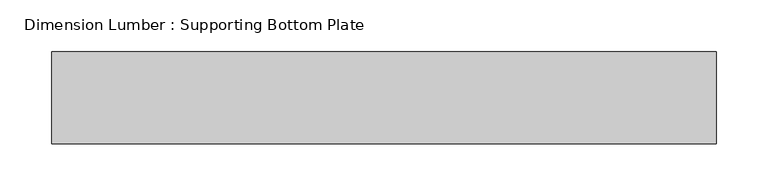
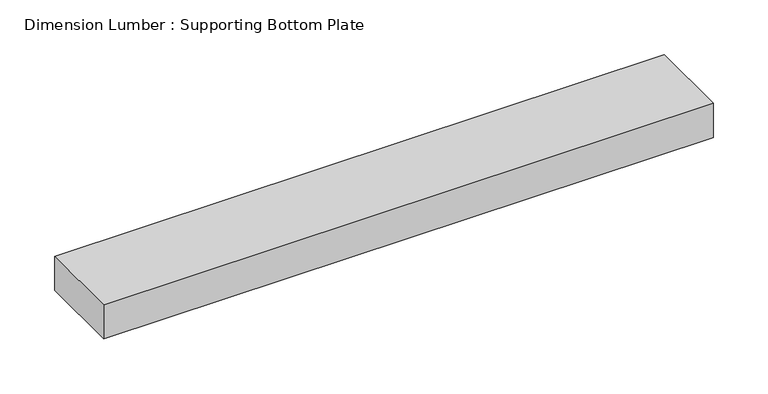
"""IFC4 building model written with IfcOpenShell, lengths in millimetres: beam geometry, Dimension Lumber : Supporting Bottom Plate."""

import ifcopenshell
import ifcopenshell.guid

model = None  # the IFC model being written
_history = None  # IfcOwnerHistory: only IFC2X3 demands one
_inside = {}  # id of a spatial element -> (the spatial element, [elements in it])
_under = {}  # id of a project, library or spatial element -> (it, [spatial elements below it])
_declared = {}  # id of a project -> (the project, [libraries it declares])
_typed = {}  # id of a type object -> (the type object, [elements of that type])
_made_of = {}  # id of a material, layer set ... -> (it, [elements and type objects made of it])


def new_model(schema):
    """Start an empty IFC model of exactly this schema.

    Asked for "IFC4X3", IfcOpenShell would pick the latest addendum, in which some entities
    have other attributes; the version numbers below select the first issue.
    IFC2X3 requires an IfcOwnerHistory on every rooted entity: one is made here for all.
    """
    global model, _history
    if schema == "IFC4X3":
        model = ifcopenshell.file(schema_version=(4, 3, 0, 0))
    else:
        model = ifcopenshell.file(schema=schema)
    _inside.clear()
    _under.clear()
    _declared.clear()
    _typed.clear()
    _made_of.clear()
    _history = None
    if model.schema == "IFC2X3":
        org = make("IfcOrganization", Name="unknown")
        user = make(
            "IfcPersonAndOrganization",
            ThePerson=make("IfcPerson", FamilyName="unknown"),
            TheOrganization=org,
        )
        app = make(
            "IfcApplication",
            ApplicationDeveloper=org,
            Version="unknown",
            ApplicationFullName="unknown",
            ApplicationIdentifier="unknown",
        )
        _history = make(
            "IfcOwnerHistory",
            OwningUser=user,
            OwningApplication=app,
            ChangeAction="ADDED",
            CreationDate=0,
        )
    return model


def make(cls, **values):
    """One entity of the class cls with the attributes given. An attribute that is None is left unset."""
    return model.create_entity(
        cls, **{name: value for name, value in values.items() if value is not None}
    )


def rooted(cls, **values):
    """An entity with a GlobalId (a new one), such as an element, a storey or a relation."""
    return make(cls, GlobalId=ifcopenshell.guid.new(), OwnerHistory=_history, **values)


def si_unit(unit_type, name, prefix=None):
    """IfcSIUnit, for example si_unit("LENGTHUNIT", "METRE", prefix="MILLI")."""
    return make("IfcSIUnit", UnitType=unit_type, Prefix=prefix, Name=name)


def assignment(units):
    """IfcUnitAssignment: the units of a project."""
    return None if units is None else make("IfcUnitAssignment", Units=units)


def point(xyz):
    """IfcCartesianPoint."""
    return None if xyz is None else make("IfcCartesianPoint", Coordinates=xyz)


def direction(xyz):
    """IfcDirection."""
    return None if xyz is None else make("IfcDirection", DirectionRatios=xyz)


def frame(location, z_axis=None, x_axis=None):
    """IfcAxis2Placement3D, a coordinate frame: its origin and axes. An axis left out is left unset."""
    return make(
        "IfcAxis2Placement3D",
        Location=point(location),
        Axis=direction(z_axis),
        RefDirection=direction(x_axis),
    )


def origin():
    """The frame at (0, 0, 0) with its axes left unset."""
    return frame((0.0, 0.0, 0.0))


def place(relative_to, where):
    """IfcLocalPlacement: puts the frame where relative to a parent placement (None: the world)."""
    return make(
        "IfcLocalPlacement", PlacementRelTo=relative_to, RelativePlacement=where
    )


def context(
    kind, dimensions, precision=None, world=None, true_north=None, identifier=None
):
    """IfcGeometricRepresentationContext, for example the 3D "Model" context."""
    return make(
        "IfcGeometricRepresentationContext",
        ContextIdentifier=identifier,
        ContextType=kind,
        CoordinateSpaceDimension=dimensions,
        Precision=precision,
        WorldCoordinateSystem=world,
        TrueNorth=true_north,
    )


def project(units=None, contexts=None):
    """IfcProject with its units and contexts."""
    return rooted(
        "IfcProject",
        Name="project",
        RepresentationContexts=contexts,
        UnitsInContext=assignment(units),
    )


def spatial(cls, under=None, at=None, **own):
    """A site, building, storey or space (cls), placed at a placement, below another one or the project."""
    s = rooted(cls, ObjectPlacement=at, **own)
    if under is not None:
        _under.setdefault(under.id(), (under, []))[1].append(s)
    return s


def polyline(points):
    """IfcPolyline through the points."""
    return make("IfcPolyline", Points=[point(p) for p in points])


def outline(outer, holes=None, kind="AREA"):
    """IfcArbitraryClosedProfileDef: a profile drawn as a closed curve; with holes, ...WithVoids."""
    if holes is None:
        return make("IfcArbitraryClosedProfileDef", ProfileType=kind, OuterCurve=outer)
    return make(
        "IfcArbitraryProfileDefWithVoids",
        ProfileType=kind,
        OuterCurve=outer,
        InnerCurves=holes,
    )


def extrude(swept, where, along, depth):
    """IfcExtrudedAreaSolid: the profile swept, set in the frame where, extruded along a direction by depth."""
    return make(
        "IfcExtrudedAreaSolid",
        SweptArea=swept,
        Position=where,
        ExtrudedDirection=direction(along),
        Depth=depth,
    )


def shape(context_of_items, identifier, shape_type, items):
    """IfcShapeRepresentation: the items that make up one representation, for example the "Body"."""
    return make(
        "IfcShapeRepresentation",
        ContextOfItems=context_of_items,
        RepresentationIdentifier=identifier,
        RepresentationType=shape_type,
        Items=items,
    )


def source(mapping_origin, context_of_items, identifier, shape_type, items):
    """IfcRepresentationMap: a shape defined once, which mapped items show again and again."""
    return make(
        "IfcRepresentationMap",
        MappingOrigin=mapping_origin,
        MappedRepresentation=shape(context_of_items, identifier, shape_type, items),
    )


def transform(
    local_origin,
    x_axis=None,
    y_axis=None,
    z_axis=None,
    scale=None,
    scale2=None,
    scale3=None,
    uniform=True,
):
    """IfcCartesianTransformationOperator3D, or its non-uniform kind. x_axis, y_axis, z_axis: its Axis1, 2, 3."""
    if uniform:
        return make(
            "IfcCartesianTransformationOperator3D",
            Axis1=direction(x_axis),
            Axis2=direction(y_axis),
            LocalOrigin=point(local_origin),
            Scale=scale,
            Axis3=direction(z_axis),
        )
    return make(
        "IfcCartesianTransformationOperator3DnonUniform",
        Axis1=direction(x_axis),
        Axis2=direction(y_axis),
        LocalOrigin=point(local_origin),
        Scale=scale,
        Axis3=direction(z_axis),
        Scale2=scale2,
        Scale3=scale3,
    )


def mapped(mapping_source, mapping_target):
    """IfcMappedItem: shows the shape of a source again, moved by a transform."""
    return make(
        "IfcMappedItem", MappingSource=mapping_source, MappingTarget=mapping_target
    )


def made_of(thing, what):
    """Note that an element or type object is made of a material, layer set ...; save() writes the relation."""
    if what is not None:
        _made_of.setdefault(what.id(), (what, []))[1].append(thing)
    return thing


def element(
    cls,
    number,
    at=None,
    inside=None,
    cuts=None,
    type_object=None,
    material=None,
    context=None,
    identifier="Body",
    shape_type=None,
    held_by="IfcProductDefinitionShape",
    body=None,
    shapes=None,
    **own,
):
    """One element of the class cls, such as IfcWall. Its Tag is "e" and its number.

    at: its placement. inside: the storey or other place that contains it. cuts: it is an
    opening in that element (IfcRelVoidsElement). A single representation is given by context,
    identifier, shape_type and body (its items); several are given by shapes. held_by: the class
    of the entity that holds the representations. save() writes the other relations.
    """
    e = rooted(cls, Tag="e%d" % number, ObjectPlacement=at, **own)
    if body is not None:
        shapes = [shape(context, identifier, shape_type, body)]
    if shapes is not None:
        e.Representation = make(held_by, Representations=shapes)
    if inside is not None:
        _inside.setdefault(inside.id(), (inside, []))[1].append(e)
    if cuts is not None:
        rooted(
            "IfcRelVoidsElement", RelatingBuildingElement=cuts, RelatedOpeningElement=e
        )
    if type_object is not None:
        _typed.setdefault(type_object.id(), (type_object, []))[1].append(e)
    return made_of(e, material)


def aggregate(whole, parts):
    """IfcRelAggregates: a whole, such as a stair, and the parts it consists of."""
    return rooted("IfcRelAggregates", RelatingObject=whole, RelatedObjects=parts)


def save(model, path):
    """Write the relations noted so far, then the file.

    IfcRelAggregates (storeys below a building ...), IfcRelContainedInSpatialStructure (elements
    in a storey), IfcRelDefinesByType, IfcRelAssociatesMaterial and IfcRelDeclares: one each for
    every whole, place, type object, material and project.
    """
    for whole, parts in _under.values():
        aggregate(whole, parts)
    for where, things in _inside.values():
        rooted(
            "IfcRelContainedInSpatialStructure",
            RelatedElements=things,
            RelatingStructure=where,
        )
    for kind, things in _typed.values():
        rooted("IfcRelDefinesByType", RelatedObjects=things, RelatingType=kind)
    for what, things in _made_of.values():
        rooted("IfcRelAssociatesMaterial", RelatedObjects=things, RelatingMaterial=what)
    for by, libraries in _declared.values():
        rooted("IfcRelDeclares", RelatingContext=by, RelatedDefinitions=libraries)
    model.write(path)


def dimension_lumber_supporting_bottom_plate_50cface6(model_context):
    return source(origin(), model_context, "Body", "SweptSolid", [
        extrude(outline(polyline([(320.675, 44.45), (320.675, -44.45), (-320.675, -44.45), (-320.675, 44.45), (320.675, 44.45)])), frame((0.0, 0.0, -19.05), z_axis=(0.0, 0.0, 1.0), x_axis=(1.0, 0.0, 0.0)), (0.0, 0.0, 1.0), 38.1),
    ])


if __name__ == "__main__":
    model = new_model("IFC4")
    model_context = context("Model", 3, world=origin())
    ifc_project = project(units=[si_unit("LENGTHUNIT", "METRE", prefix="MILLI")], contexts=[model_context])
    site = spatial("IfcSite", under=ifc_project)
    building = spatial("IfcBuilding", under=site)
    placement = place(None, origin())
    dimension_lumber_supporting_bottom_plate_shape = dimension_lumber_supporting_bottom_plate_50cface6(model_context)
    element("IfcBeam", 1, ObjectType="Dimension Lumber : Supporting Bottom Plate", at=placement, inside=building, context=model_context, shape_type="MappedRepresentation", body=[
        mapped(dimension_lumber_supporting_bottom_plate_shape, transform((0.0, 0.0, 0.0), x_axis=(1.0, 0.0, 0.0), y_axis=(0.0, 1.0, 0.0), z_axis=(0.0, 0.0, 1.0))),
    ])
    save(model, "model.ifc")

# Revit data of these elements
# Type "Dimension Lumber : Supporting Bottom Plate"
#   Assembly Code = "B10"
#   A = 0.0364583 SF
#   Length [instance default] = 5' - 0"
#   b = 0' - 3 1/2"
#   d = 0' - 1 1/2"
#   Structural Material [instance default] = Softwood, Lumber
# Element 1 (IfcBeam, "Dimension Lumber : Supporting Bottom Plate")
#   Structural Material = Douglas Fir #2
#   Materials on its faces: "Douglas Fir #2"
# Materials
#   "Softwood, Lumber": class "Wood", colour RGB 223 192 134, transparency 0, Description = "Pinus Echinata", Cost = 0
#   "Douglas Fir #2": class "Wood", colour RGB 223 192 134, transparency 0, Description = "Pinus Echinata", Cost = 0
